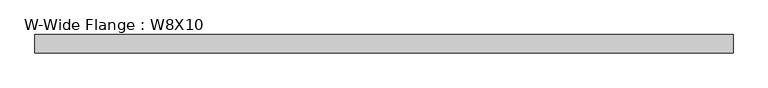
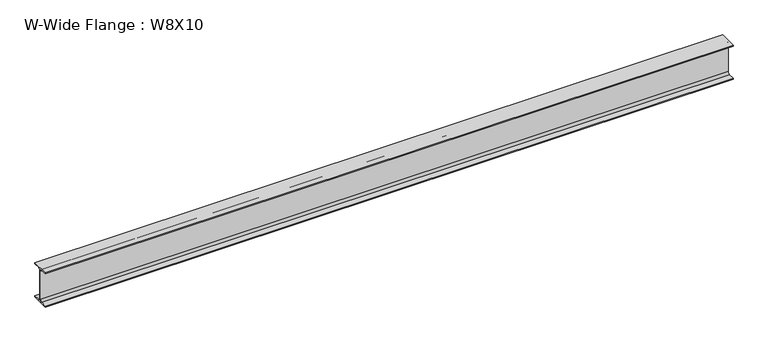
"""IFC4 building model written with IfcOpenShell, lengths in millimetres: beam geometry, W-Wide Flange : W8X10."""

from ifc_helpers import new_model, si_unit, point, frame, frame_2d, origin, place, context, project, spatial, polyline, circle_curve, trimmed, segment, composite_curve, outline, extrude, source, transform, mapped, element, save


def w_wide_flange_w8x10_1bc876d9(model_context):
    return source(origin(), model_context, "Body", "SweptSolid", [
        extrude(outline(composite_curve([segment(polyline([(50.038, -94.996), (50.038, -100.203), (-50.038, -100.203), (-50.038, -94.996), (-14.4145, -94.996)]), True, "CONTINUOUS"), segment(trimmed(circle_curve(frame_2d((-14.4145, -82.7405)), 12.2555), [point((-14.4145, -94.996))], [point((-2.159, -82.7405))], True, "CARTESIAN"), True, "CONTINUOUS"), segment(polyline([(-2.159, -82.7405), (-2.159, 82.7405)]), True, "CONTINUOUS"), segment(trimmed(circle_curve(frame_2d((-14.4145, 82.7405)), 12.2555), [point((-2.159, 82.7405))], [point((-14.4145, 94.996))], True, "CARTESIAN"), True, "CONTINUOUS"), segment(polyline([(-14.4145, 94.996), (-50.038, 94.996), (-50.038, 100.203), (50.038, 100.203), (50.038, 94.996), (14.4145, 94.996)]), True, "CONTINUOUS"), segment(trimmed(circle_curve(frame_2d((14.4145, 82.7405)), 12.2555), [point((14.4145, 94.996))], [point((2.159, 82.7405))], True, "CARTESIAN"), True, "CONTINUOUS"), segment(polyline([(2.159, 82.7405), (2.159, -82.7405)]), True, "CONTINUOUS"), segment(trimmed(circle_curve(frame_2d((14.4145, -82.7405)), 12.2555), [point((2.159, -82.7405))], [point((14.4145, -94.996))], True, "CARTESIAN"), True, "CONTINUOUS"), segment(polyline([(14.4145, -94.996), (50.038, -94.996)]), True, "CONTINUOUS")], self_intersect=False)), frame((-1916.0628906, 0.0, 0.0), z_axis=(1.0, 0.0, 0.0), x_axis=(0.0, 1.0, 0.0)), (0.0, 0.0, 1.0), 3832.1257812),
    ])


if __name__ == "__main__":
    model = new_model("IFC4")
    model_context = context("Model", 3, world=origin())
    ifc_project = project(units=[si_unit("LENGTHUNIT", "METRE", prefix="MILLI")], contexts=[model_context])
    site = spatial("IfcSite", under=ifc_project)
    building = spatial("IfcBuilding", under=site)
    placement = place(None, origin())
    w_wide_flange_w8x10_shape = w_wide_flange_w8x10_1bc876d9(model_context)
    element("IfcBeam", 1, ObjectType="W-Wide Flange : W8X10", at=placement, inside=building, context=model_context, shape_type="MappedRepresentation", body=[
        mapped(w_wide_flange_w8x10_shape, transform((0.0, 0.0, 0.0), x_axis=(1.0, 0.0, 0.0), y_axis=(0.0, 1.0, 0.0), z_axis=(0.0, 0.0, 1.0))),
    ])
    save(model, "model.ifc")

# Revit data of these elements
# Type "W-Wide Flange : W8X10"
#   Assembly Code = "B10"
#   W = 10
#   Length [instance default] = 1524 mm
#   bf = 100.076 mm
#   d = 200.406 mm
#   k = 17.463 mm
#   k2 = 12.255 mm
#   tf = 5.207 mm
#   tw = 4.318 mm
#   A = 0.00190967 m²
#   Structural Material [instance default] = Steel ASTM A992
# Element 1 (IfcBeam, "W-Wide Flange : W8X10")
#   Structural Material = Aluminum, Anodized Red
#   Materials on its faces: "Aluminum, Anodized Red"
# Materials
#   "Steel ASTM A992": class "Metal", colour RGB 128 0 0, transparency 0, Description = "Structural steel 50ksi", Cost = 0
#   "Aluminum, Anodized Red": class "Metal", colour RGB 120 120 120, transparency 0, Description = "Anodized aluminum, red", Cost = 0
